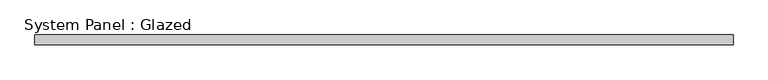
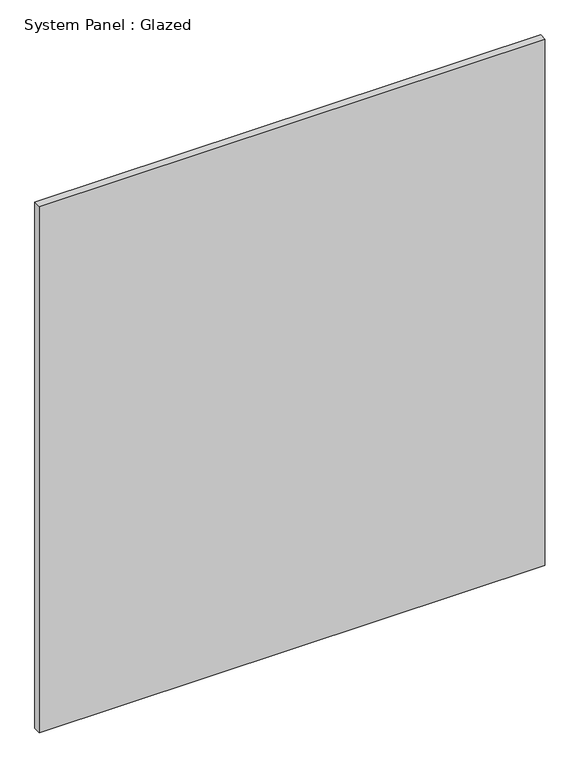
"""IFC4 building model written with IfcOpenShell, lengths in millimetres: plate geometry, System Panel : Glazed."""

from ifc_helpers import new_model, si_unit, origin, origin_with_axes, place, context, project, spatial, polyline, outline, extrude, source, transform, mapped, element, save


def system_panel_glazed_6bd6e4aa(model_context):
    return source(origin(), model_context, "Body", "SweptSolid", [
        extrude(outline(polyline([(874.2727273, 24.5), (-874.2727273, 24.5), (-874.2727273, 49.5), (874.2727273, 49.5), (874.2727273, 24.5)])), origin_with_axes(), (0.0, 0.0, 1.0), 1925.0),
    ])


if __name__ == "__main__":
    model = new_model("IFC4")
    model_context = context("Model", 3, world=origin())
    ifc_project = project(units=[si_unit("LENGTHUNIT", "METRE", prefix="MILLI")], contexts=[model_context])
    site = spatial("IfcSite", under=ifc_project)
    building = spatial("IfcBuilding", under=site)
    placement = place(None, origin())
    system_panel_glazed_shape = system_panel_glazed_6bd6e4aa(model_context)
    element("IfcPlate", 1, ObjectType="System Panel : Glazed", at=placement, inside=building, context=model_context, shape_type="MappedRepresentation", body=[
        mapped(system_panel_glazed_shape, transform((0.0, 0.0, 0.0), x_axis=(1.0, 0.0, 0.0), y_axis=(0.0, 1.0, 0.0), z_axis=(0.0, 0.0, 1.0))),
    ])
    save(model, "model.ifc")

# Revit data of these elements
# Element 1 (IfcPlate, "System Panel : Glazed")
#   Materials on its faces: "Glass"
# Materials
#   "Glass": class "Glass", colour RGB 218 227 224, transparency 0.85, Description = "Soda Lime Glass", Cost = 0
